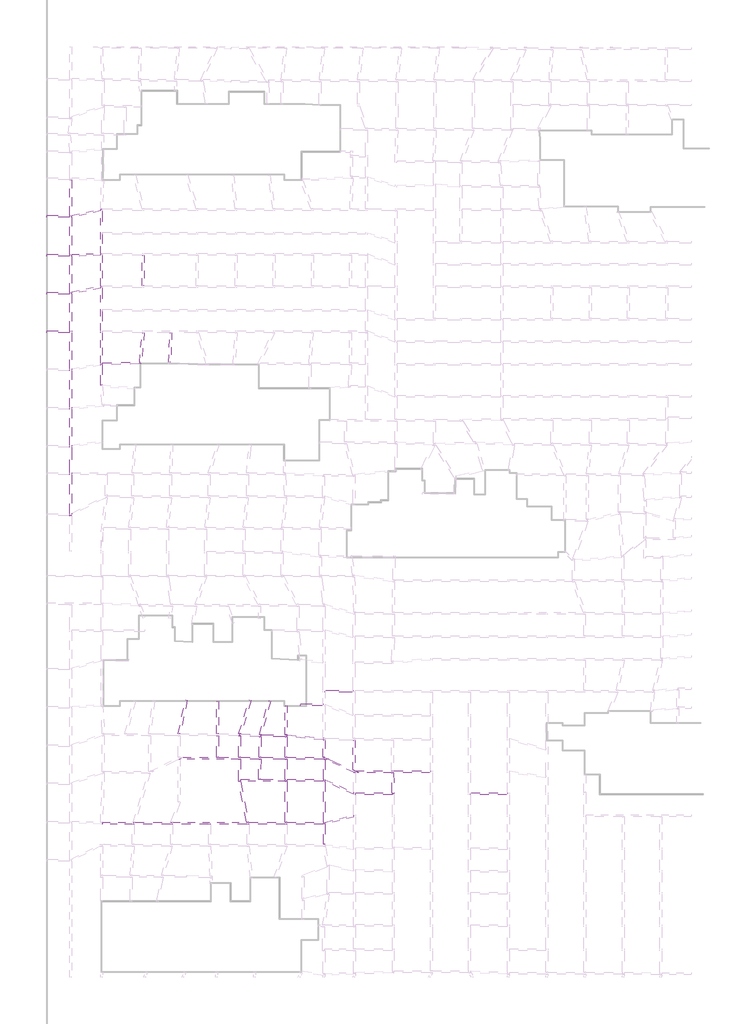
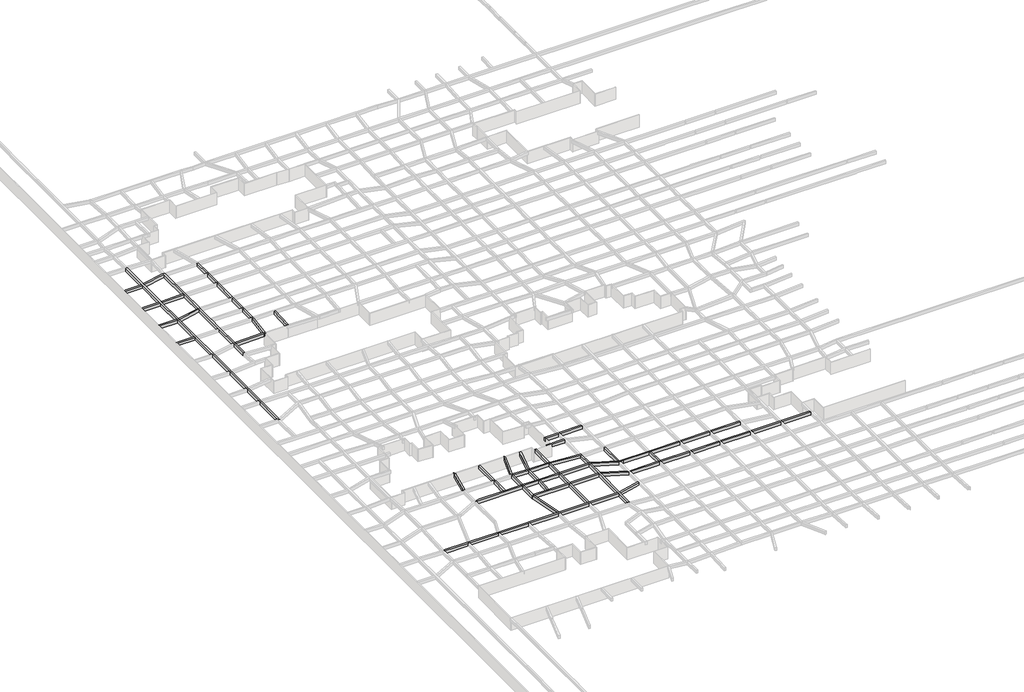
# One storey, part 26 of 45: 46 beams.
"""IFC4 building model written with IfcOpenShell, lengths in millimetres."""

from ifc_helpers import new_model, si_unit, frame, origin, place, context, project, spatial, polyline, outline, extrude, faceted_brep, element, save

model = new_model("IFC4")

# Units and contexts
model_context = context("Model", 3, world=origin())
ifc_project = project(units=[si_unit("LENGTHUNIT", "METRE", prefix="MILLI")], contexts=[model_context])

# Site, building, storey
site = spatial("IfcSite", under=ifc_project)
building = spatial("IfcBuilding", under=site)
storey = spatial("IfcBuildingStorey", under=building, Name="户型图", Elevation=0.0)

# Beams
placement = place(None, origin())
element("IfcBeam", 1, ObjectType="混凝土 - 矩形梁 : KL_beam", at=placement, inside=storey, context=model_context, shape_type="Brep", body=[
    faceted_brep([(-150359.8528414, 63929.9626201, 3300.0), (-150112.1714971, 63929.9626201, 3300.0), (-149959.8528414, 63929.9626201, 3300.0), (-149959.8528414, 64007.5728516, 3300.0), (-149959.8528414, 64456.5033467, 3300.0), (-149959.8528414, 72229.932653, 3300.0), (-149959.8528414, 72629.932653, 3300.0), (-149959.8528414, 77856.1223033, 3300.0), (-149959.8528414, 78260.0533323, 3300.0), (-149959.8528414, 85546.6664182, 3300.0), (-149959.8528414, 85948.1943532, 3300.0), (-149959.8528414, 93365.130378, 3300.0), (-149959.8528414, 93772.617056, 3300.0), (-149959.8528414, 101129.932653, 3300.0), (-149959.8528414, 101529.932653, 3300.0), (-149959.8528414, 108967.3783069, 3300.0), (-149959.8528414, 109376.0042036, 3300.0), (-149959.8528414, 116635.7245612, 3300.0), (-149959.8528414, 117035.8972944, 3300.0), (-149959.8528414, 124568.9031862, 3300.0), (-149959.8528414, 124978.3343946, 3300.0), (-149959.8528414, 132222.8565574, 3300.0), (-150162.4857077, 132229.932653, 3300.0), (-150359.8528414, 132229.932653, 3300.0), (-150359.8528414, 124929.932653, 3300.0), (-150359.8528414, 124529.932653, 3300.0), (-150359.8528414, 117029.932653, 3300.0), (-150359.8528414, 116629.932653, 3300.0), (-150359.8528414, 109329.932653, 3300.0), (-150359.8528414, 108929.932653, 3300.0), (-150359.8528414, 101529.932653, 3300.0), (-150359.8528414, 101129.932653, 3300.0), (-150359.8528414, 93729.932653, 3300.0), (-150359.8528414, 93329.932653, 3300.0), (-150359.8528414, 85929.932653, 3300.0), (-150359.8528414, 85529.932653, 3300.0), (-150359.8528414, 78229.932653, 3300.0), (-150359.8528414, 77829.932653, 3300.0), (-150359.8528414, 72629.932653, 3300.0), (-150359.8528414, 72229.932653, 3300.0), (-150359.8528414, 64329.9626201, 3300.0), (-150359.8528414, 63929.9626201, 2500.0), (-150359.8528414, 132229.932653, 2500.0), (-150359.8528414, 124929.932653, 2500.0), (-150359.8528414, 124529.932653, 2500.0), (-150359.8528414, 117029.932653, 2500.0), (-150359.8528414, 116629.932653, 2500.0), (-150359.8528414, 109329.932653, 2500.0), (-150359.8528414, 108929.932653, 2500.0), (-150359.8528414, 101529.932653, 2500.0), (-150359.8528414, 101129.932653, 2500.0), (-150359.8528414, 93729.932653, 2500.0), (-150359.8528414, 93329.932653, 2500.0), (-150359.8528414, 85929.932653, 2500.0), (-150359.8528414, 85529.932653, 2500.0), (-150359.8528414, 78229.932653, 2500.0), (-150359.8528414, 77829.932653, 2500.0), (-150359.8528414, 72629.932653, 2500.0), (-150359.8528414, 72229.932653, 2500.0), (-150359.8528414, 64329.9626201, 2500.0), (-149959.8528414, 63929.9626201, 2500.0), (-150112.1714971, 63929.9626201, 2500.0), (-150162.4857077, 132229.932653, 2500.0), (-149959.8528414, 132222.8565574, 2500.0), (-149959.8528414, 124978.3343946, 2500.0), (-149959.8528414, 124568.9031862, 2500.0), (-149959.8528414, 117035.8972944, 2500.0), (-149959.8528414, 116635.7245612, 2500.0), (-149959.8528414, 109376.0042036, 2500.0), (-149959.8528414, 108967.3783069, 2500.0), (-149959.8528414, 101529.932653, 2500.0), (-149959.8528414, 101129.932653, 2500.0), (-149959.8528414, 93772.617056, 2500.0), (-149959.8528414, 93365.130378, 2500.0), (-149959.8528414, 85948.1943532, 2500.0), (-149959.8528414, 85546.6664182, 2500.0), (-149959.8528414, 78260.0533323, 2500.0), (-149959.8528414, 77856.1223033, 2500.0), (-149959.8528414, 72629.932653, 2500.0), (-149959.8528414, 72229.932653, 2500.0), (-149959.8528414, 64456.5033467, 2500.0), (-149959.8528414, 64007.5728516, 2500.0)], [[[0, 1, 2, 3, 4, 5, 6, 7, 8, 9, 10, 11, 12, 13, 14, 15, 16, 17, 18, 19, 20, 21, 22, 23, 24, 25, 26, 27, 28, 29, 30, 31, 32, 33, 34, 35, 36, 37, 38, 39, 40]], [[41, 0, 40, 39, 38, 37, 36, 35, 34, 33, 32, 31, 30, 29, 28, 27, 26, 25, 24, 23, 42, 43, 44, 45, 46, 47, 48, 49, 50, 51, 52, 53, 54, 55, 56, 57, 58, 59]], [[60, 61, 41, 59, 58, 57, 56, 55, 54, 53, 52, 51, 50, 49, 48, 47, 46, 45, 44, 43, 42, 62, 63, 64, 65, 66, 67, 68, 69, 70, 71, 72, 73, 74, 75, 76, 77, 78, 79, 80, 81]], [[63, 21, 20, 19, 18, 17, 16, 15, 14, 13, 12, 11, 10, 9, 8, 7, 6, 5, 4, 3, 2, 60, 81, 80, 79, 78, 77, 76, 75, 74, 73, 72, 71, 70, 69, 68, 67, 66, 65, 64]], [[21, 63, 62, 22]], [[23, 22, 62, 42]], [[2, 1, 0, 41, 61, 60]]]),
])
element("IfcBeam", 2, ObjectType="混凝土 - 矩形梁 : KL_beam", at=placement, inside=storey, context=model_context, shape_type="SweptSolid", body=[
    extrude(outline(polyline([(-155040.1872489, 124529.932653), (-155040.1872489, 124929.932653), (-150359.8528414, 124929.932653), (-150359.8528414, 124529.932653), (-155040.1872489, 124529.932653)])), frame((0.0, 0.0, 2500.0), z_axis=(0.0, 0.0, 1.0), x_axis=(1.0, 0.0, 0.0)), (0.0, 0.0, 1.0), 800.0),
])
element("IfcBeam", 3, ObjectType="混凝土 - 矩形梁 : KL_beam", at=placement, inside=storey, context=model_context, shape_type="SweptSolid", body=[
    extrude(outline(polyline([(-155040.1872489, 116629.932653), (-155040.1872489, 117029.932653), (-150359.8528414, 117029.932653), (-150359.8528414, 116629.932653), (-155040.1872489, 116629.932653)])), frame((0.0, 0.0, 2500.0), z_axis=(0.0, 0.0, 1.0), x_axis=(1.0, 0.0, 0.0)), (0.0, 0.0, 1.0), 800.0),
])
element("IfcBeam", 4, ObjectType="混凝土 - 矩形梁 : KL_beam", at=placement, inside=storey, context=model_context, shape_type="SweptSolid", body=[
    extrude(outline(polyline([(-155040.1872489, 108929.932653), (-155040.1872489, 109329.932653), (-150359.8528414, 109329.932653), (-150359.8528414, 108929.932653), (-155040.1872489, 108929.932653)])), frame((0.0, 0.0, 2500.0), z_axis=(0.0, 0.0, 1.0), x_axis=(1.0, 0.0, 0.0)), (0.0, 0.0, 1.0), 800.0),
])
element("IfcBeam", 5, ObjectType="混凝土 - 矩形梁 : KL_beam", at=placement, inside=storey, context=model_context, shape_type="SweptSolid", body=[
    extrude(outline(polyline([(-155040.1872489, 101129.932653), (-155040.1872489, 101529.932653), (-150359.8528414, 101529.932653), (-150359.8528414, 101129.932653), (-155040.1872489, 101129.932653)])), frame((0.0, 0.0, 2500.0), z_axis=(0.0, 0.0, 1.0), x_axis=(1.0, 0.0, 0.0)), (0.0, 0.0, 1.0), 800.0),
])
element("IfcBeam", 6, ObjectType="混凝土 - 矩形梁 : KL_beam", at=placement, inside=storey, context=model_context, shape_type="Brep", body=[
    faceted_brep([(-144133.590805, 126250.9688143, 3300.0), (-144133.590805, 125841.5376059, 3300.0), (-144133.590805, 117207.1391417, 3300.0), (-144133.590805, 116806.9664084, 3300.0), (-144133.590805, 110592.4869991, 3300.0), (-144133.590805, 110183.8611024, 3300.0), (-144133.590805, 101529.932653, 3300.0), (-144133.590805, 101129.932653, 3300.0), (-144133.590805, 94905.1276718, 3300.0), (-144133.590805, 94497.6409938, 3300.0), (-144133.590805, 90443.9102418, 3300.0), (-143749.2394727, 90477.5366261, 3300.0), (-143733.590805, 90476.4423647, 3300.0), (-143733.590805, 94545.5936478, 3300.0), (-143733.590805, 94945.7388373, 3300.0), (-143733.590805, 101129.932653, 3300.0), (-143733.590805, 101529.932653, 3300.0), (-143733.590805, 105423.4823743, 3300.0), (-143733.590805, 105823.4823743, 3300.0), (-143733.590805, 110229.932653, 3300.0), (-143733.590805, 110629.932653, 3300.0), (-143733.590805, 116812.9362228, 3300.0), (-143733.590805, 117212.9362228, 3300.0), (-143733.590805, 121089.9393475, 3300.0), (-143733.590805, 121489.9393475, 3300.0), (-143733.590805, 125889.9393475, 3300.0), (-143733.590805, 126001.9198071, 3300.0), (-143733.590805, 126250.9688143, 3300.0), (-144087.2760394, 126250.9688143, 3300.0), (-143733.590805, 126250.9688143, 2500.0), (-143733.590805, 90476.4423647, 2500.0), (-143733.590805, 94545.5936478, 2500.0), (-143733.590805, 94945.7388373, 2500.0), (-143733.590805, 101129.932653, 2500.0), (-143733.590805, 101529.932653, 2500.0), (-143733.590805, 105423.4823743, 2500.0), (-143733.590805, 105823.4823743, 2500.0), (-143733.590805, 110229.932653, 2500.0), (-143733.590805, 110629.932653, 2500.0), (-143733.590805, 116812.9362228, 2500.0), (-143733.590805, 117212.9362228, 2500.0), (-143733.590805, 121089.9393475, 2500.0), (-143733.590805, 121489.9393475, 2500.0), (-143733.590805, 125889.9393475, 2500.0), (-143733.590805, 126001.9198071, 2500.0), (-144133.590805, 90443.9102418, 2500.0), (-144133.590805, 94497.6409938, 2500.0), (-144133.590805, 94905.1276718, 2500.0), (-144133.590805, 101129.932653, 2500.0), (-144133.590805, 101529.932653, 2500.0), (-144133.590805, 110183.8611024, 2500.0), (-144133.590805, 110592.4869991, 2500.0), (-144133.590805, 116806.9664084, 2500.0), (-144133.590805, 117207.1391417, 2500.0), (-144133.590805, 125841.5376059, 2500.0), (-144133.590805, 126250.9688143, 2500.0), (-144087.2760394, 126250.9688143, 2500.0), (-143749.2394727, 90477.5366261, 2500.0)], [[[0, 1, 2, 3, 4, 5, 6, 7, 8, 9, 10, 11, 12, 13, 14, 15, 16, 17, 18, 19, 20, 21, 22, 23, 24, 25, 26, 27, 28]], [[29, 27, 26, 25, 24, 23, 22, 21, 20, 19, 18, 17, 16, 15, 14, 13, 12, 30, 31, 32, 33, 34, 35, 36, 37, 38, 39, 40, 41, 42, 43, 44]], [[45, 46, 47, 48, 49, 50, 51, 52, 53, 54, 55, 56, 29, 44, 43, 42, 41, 40, 39, 38, 37, 36, 35, 34, 33, 32, 31, 30, 57]], [[10, 9, 8, 7, 6, 5, 4, 3, 2, 1, 0, 55, 54, 53, 52, 51, 50, 49, 48, 47, 46, 45]], [[11, 10, 45, 57]], [[12, 11, 57, 30]], [[0, 28, 27, 29, 56, 55]]]),
])
element("IfcBeam", 7, ObjectType="混凝土 - 矩形梁 : KL_beam", at=placement, inside=storey, context=model_context, shape_type="SweptSolid", body=[
    extrude(outline(polyline([(-144133.590805, 126250.9688143), (-144133.590805, 125841.5376059), (-149959.8528414, 124568.9031862), (-149959.8528414, 124978.3343946), (-144133.590805, 126250.9688143)])), frame((0.0, 0.0, 2500.0), z_axis=(0.0, 0.0, 1.0), x_axis=(1.0, 0.0, 0.0)), (0.0, 0.0, 1.0), 800.0),
])
element("IfcBeam", 8, ObjectType="混凝土 - 矩形梁 : KL_beam", at=placement, inside=storey, context=model_context, shape_type="SweptSolid", body=[
    extrude(outline(polyline([(-135233.590805, 101529.932653), (-135633.590805, 101529.932653), (-135633.590805, 105423.4823743), (-135233.590805, 105423.4823743), (-135233.590805, 101529.932653)])), frame((0.0, 0.0, 2500.0), z_axis=(0.0, 0.0, 1.0), x_axis=(1.0, 0.0, 0.0)), (0.0, 0.0, 1.0), 800.0),
    extrude(outline(polyline([(-135633.590805, 125889.9393475), (-135233.590805, 125889.9393475), (-135233.590805, 121489.9393475), (-135633.590805, 121489.9393475), (-135633.590805, 125889.9393475)])), frame((0.0, 0.0, 2500.0), z_axis=(0.0, 0.0, 1.0), x_axis=(1.0, 0.0, 0.0)), (0.0, 0.0, 1.0), 800.0),
    extrude(outline(polyline([(-135633.590805, 121089.9393475), (-135233.590805, 121089.9393475), (-135233.590805, 117212.9362228), (-135633.590805, 117212.9362228), (-135633.590805, 121089.9393475)])), frame((0.0, 0.0, 2500.0), z_axis=(0.0, 0.0, 1.0), x_axis=(1.0, 0.0, 0.0)), (0.0, 0.0, 1.0), 800.0),
    extrude(outline(polyline([(-135633.590805, 116812.9362228), (-135233.590805, 116812.9362228), (-135233.590805, 110629.932653), (-135633.590805, 110629.932653), (-135633.590805, 116812.9362228)])), frame((0.0, 0.0, 2500.0), z_axis=(0.0, 0.0, 1.0), x_axis=(1.0, 0.0, 0.0)), (0.0, 0.0, 1.0), 800.0),
    extrude(outline(polyline([(-135633.590805, 110229.932653), (-135233.590805, 110229.932653), (-135233.590805, 105823.4823743), (-135633.590805, 105823.4823743), (-135633.590805, 110229.932653)])), frame((0.0, 0.0, 2500.0), z_axis=(0.0, 0.0, 1.0), x_axis=(1.0, 0.0, 0.0)), (0.0, 0.0, 1.0), 800.0),
])
element("IfcBeam", 9, ObjectType="混凝土 - 矩形梁 : KL_beam", at=placement, inside=storey, context=model_context, shape_type="SweptSolid", body=[
    extrude(outline(polyline([(-149959.8528414, 108967.3783069), (-149959.8528414, 109376.0042036), (-144133.590805, 110592.4869991), (-144133.590805, 110183.8611024), (-149959.8528414, 108967.3783069)])), frame((0.0, 0.0, 2500.0), z_axis=(0.0, 0.0, 1.0), x_axis=(1.0, 0.0, 0.0)), (0.0, 0.0, 1.0), 800.0),
])
element("IfcBeam", 10, ObjectType="混凝土 - 矩形梁 : KL_beam", at=placement, inside=storey, context=model_context, shape_type="SweptSolid", body=[
    extrude(outline(polyline([(-149959.8528414, 116635.7245612), (-149959.8528414, 117035.8972944), (-144133.590805, 117207.1391417), (-144133.590805, 116806.9664084), (-149959.8528414, 116635.7245612)])), frame((0.0, 0.0, 2500.0), z_axis=(0.0, 0.0, 1.0), x_axis=(1.0, 0.0, 0.0)), (0.0, 0.0, 1.0), 800.0),
])
element("IfcBeam", 11, ObjectType="混凝土 - 矩形梁 : KL_beam", at=placement, inside=storey, context=model_context, shape_type="SweptSolid", body=[
    extrude(outline(polyline([(-129850.782274, 95106.8917227), (-130250.5386048, 95120.8515214), (-130040.6968677, 101129.932653), (-129640.45305, 101129.932653), (-129850.782274, 95106.8917227)])), frame((0.0, 0.0, 2500.0), z_axis=(0.0, 0.0, 1.0), x_axis=(1.0, 0.0, 0.0)), (0.0, 0.0, 1.0), 800.0),
])
element("IfcBeam", 12, ObjectType="混凝土 - 矩形梁 : KL_beam", at=placement, inside=storey, context=model_context, shape_type="Brep", body=[
    faceted_brep([(-136210.1713836, 94748.3186716, 3300.0), (-135807.6946267, 94759.1637549, 3300.0), (-135250.3245702, 101129.932653, 3300.0), (-135651.8525052, 101129.932653, 3300.0), (-136175.0804904, 95149.4094155, 3300.0), (-136210.1713836, 94748.3186716, 2500.0), (-135651.8525052, 101129.932653, 2500.0), (-136175.0804904, 95149.4094155, 2500.0), (-135807.6946267, 94759.1637549, 2500.0), (-135250.3245702, 101129.932653, 2500.0)], [[[0, 1, 2, 3, 4]], [[5, 0, 4, 3, 6, 7]], [[8, 5, 7, 6, 9]], [[1, 8, 9, 2]], [[3, 2, 9, 6]], [[1, 0, 5, 8]]]),
])
element("IfcBeam", 13, ObjectType="混凝土 - 矩形梁 : KL_beam", at=placement, inside=storey, context=model_context, shape_type="SweptSolid", body=[
    extrude(outline(polyline([(-136175.0804904, 95149.4094155), (-136210.1713836, 94748.3186716), (-143733.590805, 94545.5936478), (-143733.590805, 94945.7388373), (-136175.0804904, 95149.4094155)])), frame((0.0, 0.0, 2500.0), z_axis=(0.0, 0.0, 1.0), x_axis=(1.0, 0.0, 0.0)), (0.0, 0.0, 1.0), 800.0),
])
element("IfcBeam", 14, ObjectType="混凝土 - 矩形梁 : KL_beam", at=placement, inside=storey, context=model_context, shape_type="Brep", body=[
    faceted_brep([(-115838.9400314, 19632.6251957, 3300.0), (-115849.4144, 19232.6251957, 3300.0), (-115644.2371144, 19221.8723098, 3300.0), (-111849.9331697, 19023.0212661, 3300.0), (-111449.9331697, 19002.0581544, 3300.0), (-111449.9331697, 19012.5835366, 3300.0), (-111449.9331697, 19402.6070928, 3300.0), (-111640.2950559, 19412.5835366, 3300.0), (-111801.1398842, 19421.0130568, 3300.0), (-115578.0725211, 19618.9537088, 3300.0), (-115849.4144, 19232.6251957, 2500.0), (-115644.2371144, 19221.8723098, 2500.0), (-111849.9331697, 19023.0212661, 2500.0), (-111449.9331697, 19002.0581544, 2500.0), (-115838.9400314, 19632.6251957, 2500.0), (-115578.0725211, 19618.9537088, 2500.0), (-111801.1398842, 19421.0130568, 2500.0), (-111640.2950559, 19412.5835366, 2500.0), (-111449.9331697, 19402.6070928, 2500.0), (-111449.9331697, 19012.5835366, 2500.0)], [[[0, 1, 2, 3, 4, 5, 6, 7, 8, 9]], [[1, 10, 11, 12, 13, 4, 3, 2]], [[10, 14, 15, 16, 17, 18, 19, 13, 12, 11]], [[14, 0, 9, 8, 7, 6, 18, 17, 16, 15]], [[0, 14, 10, 1]], [[6, 5, 4, 13, 19, 18]]]),
])
element("IfcBeam", 15, ObjectType="混凝土 - 矩形梁 : KL_beam", at=placement, inside=storey, context=model_context, shape_type="Brep", body=[
    faceted_brep([(-97671.9511598, 14425.3528936, 3300.0), (-98434.5356576, 14764.877387, 3300.0), (-98570.3658693, 14825.3528936, 3300.0), (-98834.5356576, 14825.3528936, 3300.0), (-106149.9331697, 14825.3528936, 3300.0), (-106549.9331697, 14825.3528936, 3300.0), (-111449.9331697, 14825.3528936, 3300.0), (-111849.9331697, 14825.3528936, 3300.0), (-115644.2371144, 14825.3528936, 3300.0), (-116044.2371144, 14825.3528936, 3300.0), (-120144.2950634, 14825.3528936, 3300.0), (-120544.2950634, 14825.3528936, 3300.0), (-127346.5820068, 14825.3528936, 3300.0), (-128166.7035435, 14425.3528936, 3300.0), (-127944.2950634, 14425.3528936, 3300.0), (-116044.2371144, 14425.3528936, 3300.0), (-115644.2371144, 14425.3528936, 3300.0), (-111857.0472867, 14425.3528936, 3300.0), (-111456.803469, 14425.3528936, 3300.0), (-106549.9331697, 14425.3528936, 3300.0), (-106149.9331697, 14425.3528936, 3300.0), (-98812.8771817, 14425.3528936, 3300.0), (-98655.388494, 14425.3528936, 3300.0), (-97671.9511598, 14425.3528936, 2500.0), (-128166.7035435, 14425.3528936, 2500.0), (-127944.2950634, 14425.3528936, 2500.0), (-116044.2371144, 14425.3528936, 2500.0), (-115644.2371144, 14425.3528936, 2500.0), (-111857.0472867, 14425.3528936, 2500.0), (-111456.803469, 14425.3528936, 2500.0), (-106549.9331697, 14425.3528936, 2500.0), (-106149.9331697, 14425.3528936, 2500.0), (-98812.8771817, 14425.3528936, 2500.0), (-98655.388494, 14425.3528936, 2500.0), (-98570.3658693, 14825.3528936, 2500.0), (-98434.5356576, 14764.877387, 2500.0), (-127346.5820068, 14825.3528936, 2500.0), (-120544.2950634, 14825.3528936, 2500.0), (-120144.2950634, 14825.3528936, 2500.0), (-116044.2371144, 14825.3528936, 2500.0), (-115644.2371144, 14825.3528936, 2500.0), (-111849.9331697, 14825.3528936, 2500.0), (-111449.9331697, 14825.3528936, 2500.0), (-106549.9331697, 14825.3528936, 2500.0), (-106149.9331697, 14825.3528936, 2500.0), (-98834.5356576, 14825.3528936, 2500.0)], [[[0, 1, 2, 3, 4, 5, 6, 7, 8, 9, 10, 11, 12, 13, 14, 15, 16, 17, 18, 19, 20, 21, 22]], [[23, 0, 22, 21, 20, 19, 18, 17, 16, 15, 14, 13, 24, 25, 26, 27, 28, 29, 30, 31, 32, 33]], [[34, 35, 23, 33, 32, 31, 30, 29, 28, 27, 26, 25, 24, 36, 37, 38, 39, 40, 41, 42, 43, 44, 45]], [[2, 34, 45, 44, 43, 42, 41, 40, 39, 38, 37, 36, 12, 11, 10, 9, 8, 7, 6, 5, 4, 3]], [[13, 12, 36, 24]], [[2, 1, 0, 23, 35, 34]]]),
])
element("IfcBeam", 16, ObjectType="混凝土 - 矩形梁 : KL_beam", at=placement, inside=storey, context=model_context, shape_type="SweptSolid", body=[
    extrude(outline(polyline([(-120544.2950634, 19232.6251957), (-120144.2950634, 19232.6251957), (-120144.2950634, 14825.3528936), (-120544.2950634, 14825.3528936), (-120544.2950634, 19232.6251957)])), frame((0.0, 0.0, 2500.0), z_axis=(0.0, 0.0, 1.0), x_axis=(1.0, 0.0, 0.0)), (0.0, 0.0, 1.0), 800.0),
])
element("IfcBeam", 17, ObjectType="混凝土 - 矩形梁 : KL_beam", at=placement, inside=storey, context=model_context, shape_type="SweptSolid", body=[
    extrude(outline(polyline([(-115644.2371144, 14825.3528936), (-116044.2371144, 14825.3528936), (-116044.2371144, 19232.6251957), (-115849.4144, 19232.6251957), (-115644.2371144, 19221.8723098), (-115644.2371144, 14825.3528936)])), frame((0.0, 0.0, 2500.0), z_axis=(0.0, 0.0, 1.0), x_axis=(1.0, 0.0, 0.0)), (0.0, 0.0, 1.0), 800.0),
])
element("IfcBeam", 18, ObjectType="混凝土 - 矩形梁 : KL_beam", at=placement, inside=storey, context=model_context, shape_type="SweptSolid", body=[
    extrude(outline(polyline([(-111849.9331697, 19023.0212661), (-111449.9331697, 19002.0581544), (-111449.9331697, 14825.3528936), (-111849.9331697, 14825.3528936), (-111849.9331697, 19023.0212661)])), frame((0.0, 0.0, 2500.0), z_axis=(0.0, 0.0, 1.0), x_axis=(1.0, 0.0, 0.0)), (0.0, 0.0, 1.0), 800.0),
])
element("IfcBeam", 19, ObjectType="混凝土 - 矩形梁 : KL_beam", at=placement, inside=storey, context=model_context, shape_type="Brep", body=[
    faceted_brep([(-111449.9331697, 19402.6070928, 3300.0), (-111449.9331697, 19012.5835366, 3300.0), (-106549.9331697, 19012.5835366, 3300.0), (-106149.9331697, 19012.5835366, 3300.0), (-106149.9331697, 19395.8497714, 3300.0), (-106149.9331697, 19412.5835366, 3300.0), (-106341.2009811, 19412.5835366, 3300.0), (-106549.9331697, 19412.5835366, 3300.0), (-111389.2880952, 19412.5835366, 3300.0), (-111640.2950559, 19412.5835366, 3300.0), (-111449.9331697, 19012.5835366, 2500.0), (-106549.9331697, 19012.5835366, 2500.0), (-106149.9331697, 19012.5835366, 2500.0), (-111449.9331697, 19402.6070928, 2500.0), (-111640.2950559, 19412.5835366, 2500.0), (-111389.2880952, 19412.5835366, 2500.0), (-106549.9331697, 19412.5835366, 2500.0), (-106341.2009811, 19412.5835366, 2500.0), (-106149.9331697, 19412.5835366, 2500.0), (-106149.9331697, 19395.8497714, 2500.0)], [[[0, 1, 2, 3, 4, 5, 6, 7, 8, 9]], [[1, 10, 11, 12, 3, 2]], [[10, 13, 14, 15, 16, 17, 18, 19, 12, 11]], [[14, 9, 8, 7, 6, 5, 18, 17, 16, 15]], [[0, 13, 10, 1]], [[13, 0, 9, 14]], [[5, 4, 3, 12, 19, 18]]]),
])
element("IfcBeam", 20, ObjectType="混凝土 - 矩形梁 : KL_beam", at=placement, inside=storey, context=model_context, shape_type="Brep", body=[
    faceted_brep([(-106149.9331697, 19012.5835366, 3300.0), (-106549.9331697, 19012.5835366, 3300.0), (-106549.9331697, 14825.3528936, 3300.0), (-106149.9331697, 14825.3528936, 3300.0), (-106149.9331697, 18994.3218363, 3300.0), (-106549.9331697, 19012.5835366, 2500.0), (-106549.9331697, 14825.3528936, 2500.0), (-106149.9331697, 19012.5835366, 2500.0), (-106149.9331697, 18994.3218363, 2500.0), (-106149.9331697, 14825.3528936, 2500.0)], [[[0, 1, 2, 3, 4]], [[1, 5, 6, 2]], [[5, 7, 8, 9, 6]], [[7, 0, 4, 3, 9, 8]], [[1, 0, 7, 5]], [[3, 2, 6, 9]]]),
])
element("IfcBeam", 21, ObjectType="混凝土 - 矩形梁 : KL_beam", at=placement, inside=storey, context=model_context, shape_type="Brep", body=[
    faceted_brep([(-106341.2009811, 19412.5835366, 3300.0), (-106549.9331697, 19430.8452368, 3300.0), (-106549.9331697, 19412.5835366, 3300.0), (-106549.9331697, 19430.8452368, 2500.0), (-106341.2009811, 19412.5835366, 2500.0), (-106549.9331697, 19412.5835366, 2500.0)], [[[0, 1, 2]], [[3, 4, 5]], [[1, 0, 4, 3]], [[5, 2, 1, 3]], [[0, 2, 5, 4]]]),
    faceted_brep([(-98447.5025342, 18320.4464741, 2500.0), (-98447.5025342, 18320.4464741, 3300.0), (-98834.5356576, 18354.3074848, 3300.0), (-106149.9331697, 18994.3218363, 3300.0), (-106149.9331697, 18994.3218363, 2500.0), (-98834.5356576, 18354.3074848, 2500.0), (-106149.9331697, 19395.8497714, 3300.0), (-106149.9331697, 19395.8497714, 2500.0), (-106149.9331697, 19012.5835366, 2500.0), (-106149.9331697, 19012.5835366, 3300.0), (-98430.038157, 18720.4464741, 3300.0), (-98430.038157, 18720.4464741, 2500.0), (-98434.5356576, 18720.8399544, 3300.0), (-98834.5356576, 18755.8354199, 3300.0), (-98834.5356576, 18755.8354199, 2500.0), (-98434.5356576, 18720.8399544, 2500.0)], [[[0, 1, 2, 3, 4, 5]], [[6, 7, 8, 4, 3, 9]], [[10, 1, 0, 11]], [[6, 9, 3, 2, 1, 10, 12, 13]], [[4, 8, 7, 14, 15, 11, 0, 5]], [[7, 6, 13, 12, 10, 11, 15, 14]]]),
])
element("IfcBeam", 22, ObjectType="混凝土 - 矩形梁 : KL_beam", at=placement, inside=storey, context=model_context, shape_type="Brep", body=[
    faceted_brep([(-92534.6339278, 11700.217385, 3300.0), (-92291.6701424, 11700.217385, 3300.0), (-91551.1965936, 11700.217385, 3300.0), (-92449.6113031, 12100.217385, 3300.0), (-92755.3337307, 12236.3337795, 3300.0), (-97671.9511598, 14425.3528936, 3300.0), (-98655.388494, 14425.3528936, 3300.0), (-98412.8771817, 14317.3799008, 3300.0), (-92691.6701424, 11770.1344124, 3300.0), (-92534.6339278, 11700.217385, 2500.0), (-98655.388494, 14425.3528936, 2500.0), (-98412.8771817, 14317.3799008, 2500.0), (-92691.6701424, 11770.1344124, 2500.0), (-91551.1965936, 11700.217385, 2500.0), (-92291.6701424, 11700.217385, 2500.0), (-97671.9511598, 14425.3528936, 2500.0), (-92755.3337307, 12236.3337795, 2500.0), (-92449.6113031, 12100.217385, 2500.0)], [[[0, 1, 2, 3, 4, 5, 6, 7, 8]], [[9, 0, 8, 7, 6, 10, 11, 12]], [[13, 14, 9, 12, 11, 10, 15, 16, 17]], [[2, 13, 17, 16, 15, 5, 4, 3]], [[6, 5, 15, 10]], [[2, 1, 0, 9, 14, 13]]]),
])
element("IfcBeam", 23, ObjectType="混凝土 - 矩形梁 : KL_beam", at=placement, inside=storey, context=model_context, shape_type="Brep", body=[
    faceted_brep([(-61385.2176693, 11700.217385, 3300.0), (-61385.2176693, 12100.217385, 3300.0), (-68859.410716, 12100.217385, 3300.0), (-68859.410716, 11700.217385, 3300.0), (-61385.2176693, 11700.217385, 2500.0), (-68859.410716, 11700.217385, 2500.0), (-61385.2176693, 12100.217385, 2500.0), (-68859.410716, 12100.217385, 2500.0)], [[[0, 1, 2, 3]], [[4, 0, 3, 5]], [[6, 4, 5, 7]], [[1, 6, 7, 2]], [[1, 0, 4, 6]], [[3, 2, 7, 5]]]),
    faceted_brep([(-91551.1965936, 11700.217385, 3300.0), (-92449.6113031, 12100.217385, 3300.0), (-92449.6113031, 12100.217385, 2500.0), (-91551.1965936, 11700.217385, 2500.0), (-76974.0592951, 12100.217385, 3300.0), (-76974.0592951, 11700.217385, 3300.0), (-76974.0592951, 11700.217385, 2500.0), (-76974.0592951, 12100.217385, 2500.0), (-84936.5912928, 11700.217385, 3300.0), (-84536.3474751, 11700.217385, 3300.0), (-84543.4535378, 12100.217385, 3300.0), (-84943.4535378, 12100.217385, 3300.0), (-92355.3337307, 12100.217385, 3300.0), (-84936.5912928, 11700.217385, 2500.0), (-84536.3474751, 11700.217385, 2500.0), (-92355.3337307, 12100.217385, 2500.0), (-84943.4535378, 12100.217385, 2500.0), (-84543.4535378, 12100.217385, 2500.0)], [[[0, 1, 2, 3]], [[4, 5, 6, 7]], [[1, 0, 8, 9, 5, 4, 10, 11, 12]], [[0, 3, 13, 14, 6, 5, 9, 8]], [[3, 2, 15, 16, 17, 7, 6, 14, 13]], [[2, 1, 12, 11, 10, 4, 7, 17, 16, 15]]]),
    faceted_brep([(-76574.0592951, 11700.217385, 3300.0), (-76574.0592951, 12100.217385, 3300.0), (-76574.0592951, 12100.217385, 2500.0), (-76574.0592951, 11700.217385, 2500.0), (-69259.410716, 12100.217385, 3300.0), (-69259.410716, 11700.217385, 3300.0), (-69259.410716, 11700.217385, 2500.0), (-69259.410716, 12100.217385, 2500.0)], [[[0, 1, 2, 3]], [[4, 5, 6, 7]], [[1, 0, 5, 4]], [[0, 3, 6, 5]], [[3, 2, 7, 6]], [[2, 1, 4, 7]]]),
])
element("IfcBeam", 24, ObjectType="混凝土 - 矩形梁 : KL_beam", at=placement, inside=storey, context=model_context, shape_type="SweptSolid", body=[
    extrude(outline(polyline([(-92691.6701424, 7708.1903778), (-92691.6701424, 7270.3358664), (-98412.8771817, 9817.5813548), (-98412.8771817, 10255.4358662), (-92691.6701424, 7708.1903778)])), frame((0.0, 0.0, 2500.0), z_axis=(0.0, 0.0, 1.0), x_axis=(1.0, 0.0, 0.0)), (0.0, 0.0, 1.0), 800.0),
])
element("IfcBeam", 25, ObjectType="混凝土 - 矩形梁 : KL_beam", at=placement, inside=storey, context=model_context, shape_type="Brep", body=[
    faceted_brep([(-98812.8771817, -2906.533538, 3300.0), (-98412.8771817, -2906.533538, 3300.0), (-98412.8771817, 1237.2093367, 3300.0), (-98412.8771817, 1649.4547885, 3300.0), (-98412.8771817, 9817.5813548, 3300.0), (-98412.8771817, 10255.4358662, 3300.0), (-98412.8771817, 14317.3799008, 3300.0), (-98655.388494, 14425.3528936, 3300.0), (-98812.8771817, 14425.3528936, 3300.0), (-98812.8771817, 10325.4890447, 3300.0), (-98812.8771817, 9925.4890447, 3300.0), (-98812.8771817, 1593.466462, 3300.0), (-98812.8771817, 1193.466462, 3300.0), (-98812.8771817, -2906.533538, 2500.0), (-98812.8771817, 14425.3528936, 2500.0), (-98812.8771817, 10325.4890447, 2500.0), (-98812.8771817, 9925.4890447, 2500.0), (-98812.8771817, 1593.466462, 2500.0), (-98812.8771817, 1193.466462, 2500.0), (-98412.8771817, -2906.533538, 2500.0), (-98655.388494, 14425.3528936, 2500.0), (-98412.8771817, 14317.3799008, 2500.0), (-98412.8771817, 10255.4358662, 2500.0), (-98412.8771817, 9817.5813548, 2500.0), (-98412.8771817, 1649.4547885, 2500.0), (-98412.8771817, 1237.2093367, 2500.0)], [[[0, 1, 2, 3, 4, 5, 6, 7, 8, 9, 10, 11, 12]], [[13, 0, 12, 11, 10, 9, 8, 14, 15, 16, 17, 18]], [[19, 13, 18, 17, 16, 15, 14, 20, 21, 22, 23, 24, 25]], [[1, 19, 25, 24, 23, 22, 21, 6, 5, 4, 3, 2]], [[1, 0, 13, 19]], [[14, 8, 7, 20]], [[7, 6, 21, 20]]]),
])
element("IfcBeam", 26, ObjectType="混凝土 - 矩形梁 : KL_beam", at=placement, inside=storey, context=model_context, shape_type="Brep", body=[
    faceted_brep([(-98812.8771817, 1193.466462, 3300.0), (-98812.8771817, 1593.466462, 3300.0), (-106150.085142, 1593.466462, 3300.0), (-106550.085142, 1593.466462, 3300.0), (-113978.3630926, 1593.466462, 3300.0), (-114385.8825203, 1593.466462, 3300.0), (-129385.5729072, 1593.466462, 3300.0), (-129809.5937678, 1593.466462, 3300.0), (-137035.6604812, 1593.466462, 3300.0), (-137453.9371838, 1593.466462, 3300.0), (-143698.467803, 1593.466462, 3300.0), (-143704.0852782, 1432.6030214, 3300.0), (-143704.0852782, 1228.9879716, 3300.0), (-143704.0852782, 1193.466462, 3300.0), (-137667.9283627, 1193.466462, 3300.0), (-137267.9283627, 1193.466462, 3300.0), (-129867.9283627, 1193.466462, 3300.0), (-129467.9283627, 1193.466462, 3300.0), (-122143.1610176, 1193.466462, 3300.0), (-121743.1610176, 1193.466462, 3300.0), (-114343.1610176, 1193.466462, 3300.0), (-113943.1610176, 1193.466462, 3300.0), (-106543.1610176, 1193.466462, 3300.0), (-106143.1610176, 1193.466462, 3300.0), (-98812.8771817, 1593.466462, 2500.0), (-106150.085142, 1593.466462, 2500.0), (-106550.085142, 1593.466462, 2500.0), (-113978.3630926, 1593.466462, 2500.0), (-114385.8825203, 1593.466462, 2500.0), (-129385.5729072, 1593.466462, 2500.0), (-129809.5937678, 1593.466462, 2500.0), (-137035.6604812, 1593.466462, 2500.0), (-137453.9371838, 1593.466462, 2500.0), (-143698.467803, 1593.466462, 2500.0), (-98812.8771817, 1193.466462, 2500.0), (-106143.1610176, 1193.466462, 2500.0), (-106543.1610176, 1193.466462, 2500.0), (-113943.1610176, 1193.466462, 2500.0), (-114343.1610176, 1193.466462, 2500.0), (-121743.1610176, 1193.466462, 2500.0), (-122143.1610176, 1193.466462, 2500.0), (-129467.9283627, 1193.466462, 2500.0), (-129867.9283627, 1193.466462, 2500.0), (-137267.9283627, 1193.466462, 2500.0), (-137667.9283627, 1193.466462, 2500.0), (-143704.0852782, 1193.466462, 2500.0), (-143704.0852782, 1228.9879716, 2500.0), (-143704.0852782, 1432.6030214, 2500.0)], [[[0, 1, 2, 3, 4, 5, 6, 7, 8, 9, 10, 11, 12, 13, 14, 15, 16, 17, 18, 19, 20, 21, 22, 23]], [[1, 24, 25, 26, 27, 28, 29, 30, 31, 32, 33, 10, 9, 8, 7, 6, 5, 4, 3, 2]], [[24, 34, 35, 36, 37, 38, 39, 40, 41, 42, 43, 44, 45, 46, 47, 33, 32, 31, 30, 29, 28, 27, 26, 25]], [[34, 0, 23, 22, 21, 20, 19, 18, 17, 16, 15, 14, 13, 45, 44, 43, 42, 41, 40, 39, 38, 37, 36, 35]], [[1, 0, 34, 24]], [[45, 13, 12, 11, 47, 46]], [[11, 10, 33, 47]]]),
])
element("IfcBeam", 27, ObjectType="混凝土 - 矩形梁 : KL_beam", at=placement, inside=storey, context=model_context, shape_type="SweptSolid", body=[
    extrude(outline(polyline([(-111857.0472867, 14425.3528936), (-111456.803469, 14425.3528936), (-111599.9738694, 10325.4890447), (-112000.2176871, 10325.4890447), (-111857.0472867, 14425.3528936)])), frame((0.0, 0.0, 2500.0), z_axis=(0.0, 0.0, 1.0), x_axis=(1.0, 0.0, 0.0)), (0.0, 0.0, 1.0), 800.0),
])
element("IfcBeam", 28, ObjectType="混凝土 - 矩形梁 : KL_beam", at=placement, inside=storey, context=model_context, shape_type="Brep", body=[
    faceted_brep([(-106549.9331697, 9925.4890447, 3300.0), (-106149.9331697, 9925.4890447, 3300.0), (-106149.9331697, 10325.4890447, 3300.0), (-106149.9331697, 14425.3528936, 3300.0), (-106549.9331697, 14425.3528936, 3300.0), (-106549.9331697, 10325.4890447, 3300.0), (-106549.9331697, 9925.4890447, 2500.0), (-106549.9331697, 14425.3528936, 2500.0), (-106549.9331697, 10325.4890447, 2500.0), (-106149.9331697, 9925.4890447, 2500.0), (-106149.9331697, 14425.3528936, 2500.0), (-106149.9331697, 10325.4890447, 2500.0)], [[[0, 1, 2, 3, 4, 5]], [[6, 0, 5, 4, 7, 8]], [[9, 6, 8, 7, 10, 11]], [[1, 9, 11, 10, 3, 2]], [[4, 3, 10, 7]], [[1, 0, 6, 9]]]),
])
element("IfcBeam", 29, ObjectType="混凝土 - 矩形梁 : KL_beam", at=placement, inside=storey, context=model_context, shape_type="Brep", body=[
    faceted_brep([(-116044.2371144, 9925.4890447, 3300.0), (-116009.0350395, 9925.4890447, 3300.0), (-115644.2371144, 9925.4890447, 3300.0), (-115644.2371144, 10325.4890447, 3300.0), (-115644.2371144, 14425.3528936, 3300.0), (-116044.2371144, 14425.3528936, 3300.0), (-116044.2371144, 9925.4890447, 2500.0), (-116044.2371144, 14425.3528936, 2500.0), (-115644.2371144, 9925.4890447, 2500.0), (-116009.0350395, 9925.4890447, 2500.0), (-115644.2371144, 14425.3528936, 2500.0), (-115644.2371144, 10325.4890447, 2500.0)], [[[0, 1, 2, 3, 4, 5]], [[6, 0, 5, 7]], [[8, 9, 6, 7, 10, 11]], [[2, 8, 11, 10, 4, 3]], [[5, 4, 10, 7]], [[2, 1, 0, 6, 9, 8]]]),
])
element("IfcBeam", 30, ObjectType="混凝土 - 矩形梁 : KL_beam", at=placement, inside=storey, context=model_context, shape_type="Brep", body=[
    faceted_brep([(-106549.9331697, 9925.4890447, 3300.0), (-106549.9331697, 10325.4890447, 3300.0), (-111599.9738694, 10325.4890447, 3300.0), (-112000.2176871, 10325.4890447, 3300.0), (-115644.2371144, 10325.4890447, 3300.0), (-115644.2371144, 9925.4890447, 3300.0), (-115601.5156118, 9925.4890447, 3300.0), (-106549.9331697, 9925.4890447, 2500.0), (-115644.2371144, 9925.4890447, 2500.0), (-115601.5156118, 9925.4890447, 2500.0), (-106549.9331697, 10325.4890447, 2500.0), (-115644.2371144, 10325.4890447, 2500.0), (-112000.2176871, 10325.4890447, 2500.0), (-111599.9738694, 10325.4890447, 2500.0)], [[[0, 1, 2, 3, 4, 5, 6]], [[7, 0, 6, 5, 8, 9]], [[10, 7, 9, 8, 11, 12, 13]], [[1, 10, 13, 12, 11, 4, 3, 2]], [[1, 0, 7, 10]], [[5, 4, 11, 8]]]),
])
element("IfcBeam", 31, ObjectType="混凝土 - 矩形梁 : KL_beam", at=placement, inside=storey, context=model_context, shape_type="SweptSolid", body=[
    extrude(outline(polyline([(-106149.9331697, 9925.4890447), (-106149.9331697, 10325.4890447), (-98812.8771817, 10325.4890447), (-98812.8771817, 9925.4890447), (-106149.9331697, 9925.4890447)])), frame((0.0, 0.0, 2500.0), z_axis=(0.0, 0.0, 1.0), x_axis=(1.0, 0.0, 0.0)), (0.0, 0.0, 1.0), 800.0),
])
element("IfcBeam", 32, ObjectType="混凝土 - 矩形梁 : KL_beam", at=placement, inside=storey, context=model_context, shape_type="SweptSolid", body=[
    extrude(outline(polyline([(-106550.085142, 9925.4890447), (-106150.085142, 9925.4890447), (-106150.085142, 1593.466462), (-106550.085142, 1593.466462), (-106550.085142, 9925.4890447)])), frame((0.0, 0.0, 2500.0), z_axis=(0.0, 0.0, 1.0), x_axis=(1.0, 0.0, 0.0)), (0.0, 0.0, 1.0), 800.0),
])
element("IfcBeam", 33, ObjectType="混凝土 - 矩形梁 : KL_beam", at=placement, inside=storey, context=model_context, shape_type="Brep", body=[
    faceted_brep([(-115601.5156118, 9925.4890447, 3300.0), (-115644.2371144, 9925.4890447, 3300.0), (-116009.0350395, 9925.4890447, 3300.0), (-114385.8825203, 1593.466462, 3300.0), (-113978.3630926, 1593.466462, 3300.0), (-116009.0350395, 9925.4890447, 2500.0), (-114385.8825203, 1593.466462, 2500.0), (-115644.2371144, 9925.4890447, 2500.0), (-115601.5156118, 9925.4890447, 2500.0), (-113978.3630926, 1593.466462, 2500.0)], [[[0, 1, 2, 3, 4]], [[2, 5, 6, 3]], [[5, 7, 8, 9, 6]], [[8, 0, 4, 9]], [[5, 2, 1, 0, 8, 7]], [[4, 3, 6, 9]]]),
])
element("IfcBeam", 34, ObjectType="混凝土 - 矩形梁 : KL_beam", at=placement, inside=storey, context=model_context, shape_type="SweptSolid", body=[
    extrude(outline(polyline([(-102355.449792, 27984.5858537), (-102355.449792, 28384.5858537), (-98834.5356576, 28384.5858537), (-98834.5356576, 27984.5858537), (-102355.449792, 27984.5858537)])), frame((0.0, 0.0, 2500.0), z_axis=(0.0, 0.0, 1.0), x_axis=(1.0, 0.0, 0.0)), (0.0, 0.0, 1.0), 800.0),
    extrude(outline(polyline([(-92755.449792, 28384.5858537), (-92755.449792, 27984.5858537), (-98434.5356576, 27984.5858537), (-98434.5356576, 28384.5858537), (-92755.449792, 28384.5858537)])), frame((0.0, 0.0, 2500.0), z_axis=(0.0, 0.0, 1.0), x_axis=(1.0, 0.0, 0.0)), (0.0, 0.0, 1.0), 800.0),
])
element("IfcBeam", 35, ObjectType="混凝土 - 矩形梁 : KL_beam", at=placement, inside=storey, context=model_context, shape_type="SweptSolid", body=[
    extrude(outline(polyline([(-103434.5356576, 25264.534172), (-103434.5356576, 25664.534172), (-98834.5356576, 25664.534172), (-98834.5356576, 25264.534172), (-103434.5356576, 25264.534172)])), frame((0.0, 0.0, 2500.0), z_axis=(0.0, 0.0, 1.0), x_axis=(1.0, 0.0, 0.0)), (0.0, 0.0, 1.0), 800.0),
])
element("IfcBeam", 36, ObjectType="混凝土 - 矩形梁 : KL_beam", at=placement, inside=storey, context=model_context, shape_type="SweptSolid", body=[
    extrude(outline(polyline([(-126850.2294704, 26482.6720173), (-126458.9704301, 26399.507341), (-127897.3156321, 19632.6251957), (-128306.2518701, 19632.6251957), (-126850.2294704, 26482.6720173)])), frame((0.0, 0.0, 2500.0), z_axis=(0.0, 0.0, 1.0), x_axis=(1.0, 0.0, 0.0)), (0.0, 0.0, 1.0), 800.0),
])
element("IfcBeam", 37, ObjectType="混凝土 - 矩形梁 : KL_beam", at=placement, inside=storey, context=model_context, shape_type="SweptSolid", body=[
    extrude(outline(polyline([(-120544.2950634, 26232.6251957), (-120144.2950634, 26232.6251957), (-120144.2950634, 19632.6251957), (-120544.2950634, 19632.6251957), (-120544.2950634, 26232.6251957)])), frame((0.0, 0.0, 2500.0), z_axis=(0.0, 0.0, 1.0), x_axis=(1.0, 0.0, 0.0)), (0.0, 0.0, 1.0), 800.0),
])
element("IfcBeam", 38, ObjectType="混凝土 - 矩形梁 : KL_beam", at=placement, inside=storey, context=model_context, shape_type="SweptSolid", body=[
    extrude(outline(polyline([(-113901.1247224, 26472.1242552), (-113518.60282, 26355.1755733), (-115578.0725211, 19618.9537088), (-115838.9400314, 19632.6251957), (-115992.1694307, 19632.6251957), (-113901.1247224, 26472.1242552)])), frame((0.0, 0.0, 2500.0), z_axis=(0.0, 0.0, 1.0), x_axis=(1.0, 0.0, 0.0)), (0.0, 0.0, 1.0), 800.0),
])
element("IfcBeam", 39, ObjectType="混凝土 - 矩形梁 : KL_beam", at=placement, inside=storey, context=model_context, shape_type="SweptSolid", body=[
    extrude(outline(polyline([(-109953.7393057, 26315.6058775), (-109567.3689752, 26212.0782594), (-111389.2880952, 19412.5835366), (-111640.2950559, 19412.5835366), (-111801.1398842, 19421.0130568), (-109953.7393057, 26315.6058775)])), frame((0.0, 0.0, 2500.0), z_axis=(0.0, 0.0, 1.0), x_axis=(1.0, 0.0, 0.0)), (0.0, 0.0, 1.0), 800.0),
])
element("IfcBeam", 40, ObjectType="混凝土 - 矩形梁 : KL_beam", at=placement, inside=storey, context=model_context, shape_type="SweptSolid", body=[
    extrude(outline(polyline([(-106549.9331697, 25288.6033534), (-106149.9331697, 25288.6033534), (-106149.9331697, 19412.5835366), (-106341.2009811, 19412.5835366), (-106549.9331697, 19430.8452368), (-106549.9331697, 25288.6033534)])), frame((0.0, 0.0, 2500.0), z_axis=(0.0, 0.0, 1.0), x_axis=(1.0, 0.0, 0.0)), (0.0, 0.0, 1.0), 800.0),
])
element("IfcBeam", 41, ObjectType="混凝土 - 矩形梁 : KL_beam", at=placement, inside=storey, context=model_context, shape_type="SweptSolid", body=[
    extrude(outline(polyline([(-92691.6701424, 3075.9119134), (-92691.6701424, 2663.6664617), (-98412.8771817, 1237.2093367), (-98412.8771817, 1649.4547885), (-92691.6701424, 3075.9119134)])), frame((0.0, 0.0, 2500.0), z_axis=(0.0, 0.0, 1.0), x_axis=(1.0, 0.0, 0.0)), (0.0, 0.0, 1.0), 800.0),
])
element("IfcBeam", 42, ObjectType="混凝土 - 矩形梁 : KL_beam", at=placement, inside=storey, context=model_context, shape_type="Brep", body=[
    faceted_brep([(-98834.5356576, 14825.3528936, 2500.0), (-98834.5356576, 14825.3528936, 3300.0), (-98834.5356576, 18354.3074848, 3300.0), (-98834.5356576, 18354.3074848, 2500.0), (-98570.3658693, 14825.3528936, 2500.0), (-98570.3658693, 14825.3528936, 3300.0), (-98812.8771817, 14825.3528936, 3300.0), (-98812.8771817, 14825.3528936, 2500.0), (-98434.5356576, 14764.877387, 2500.0), (-98434.5356576, 14764.877387, 3300.0), (-98434.5356576, 18320.4464741, 3300.0), (-98447.5025342, 18320.4464741, 3300.0), (-98447.5025342, 18320.4464741, 2500.0), (-98434.5356576, 18320.4464741, 2500.0)], [[[0, 1, 2, 3]], [[4, 5, 6, 1, 0, 7]], [[5, 4, 8, 9]], [[5, 9, 10, 11, 2, 1, 6]], [[8, 4, 7, 0, 3, 12, 13]], [[9, 8, 13, 10]], [[3, 2, 11, 12]], [[11, 10, 13, 12]]]),
])
element("IfcBeam", 43, ObjectType="混凝土 - 矩形梁 : KL_beam", at=placement, inside=storey, context=model_context, shape_type="Brep", body=[
    faceted_brep([(-92355.3337307, 18320.4464741, 3300.0), (-92755.3337307, 18320.4464741, 3300.0), (-92755.3337307, 12236.3337795, 3300.0), (-92691.6701424, 12207.9889238, 3300.0), (-92449.6113031, 12100.217385, 3300.0), (-92355.3337307, 12100.217385, 3300.0), (-92755.3337307, 18320.4464741, 2500.0), (-92755.3337307, 12236.3337795, 2500.0), (-92355.3337307, 18320.4464741, 2500.0), (-92355.3337307, 12100.217385, 2500.0), (-92449.6113031, 12100.217385, 2500.0), (-92691.6701424, 12207.9889238, 2500.0)], [[[0, 1, 2, 3, 4, 5]], [[1, 6, 7, 2]], [[6, 8, 9, 10, 11, 7]], [[8, 0, 5, 9]], [[1, 0, 8, 6]], [[2, 7, 11, 10, 4, 3]], [[5, 4, 10, 9]]]),
])
element("IfcBeam", 44, ObjectType="混凝土 - 矩形梁 : KL_beam", at=placement, inside=storey, context=model_context, shape_type="Brep", body=[
    faceted_brep([(-84786.4058027, 7399.4676504, 3300.0), (-84386.4058027, 7406.4496764, 3300.0), (-84393.1758376, 7600.318112, 3300.0), (-84536.3474751, 11700.217385, 3300.0), (-84936.5912928, 11700.217385, 3300.0), (-84793.4196553, 7600.318112, 3300.0), (-84786.4058027, 7399.4676504, 2500.0), (-84936.5912928, 11700.217385, 2500.0), (-84793.4196553, 7600.318112, 2500.0), (-84386.4058027, 7406.4496764, 2500.0), (-84536.3474751, 11700.217385, 2500.0), (-84393.1758376, 7600.318112, 2500.0)], [[[0, 1, 2, 3, 4, 5]], [[6, 0, 5, 4, 7, 8]], [[9, 6, 8, 7, 10, 11]], [[1, 9, 11, 10, 3, 2]], [[4, 3, 10, 7]], [[1, 0, 6, 9]]]),
])
element("IfcBeam", 45, ObjectType="混凝土 - 矩形梁 : KL_beam", at=placement, inside=storey, context=model_context, shape_type="SweptSolid", body=[
    extrude(outline(polyline([(-92291.6701424, 7200.318112), (-92291.6701424, 7600.318112), (-84793.4196553, 7600.318112), (-84786.4058027, 7399.4676504), (-84786.4058027, 7200.318112), (-92291.6701424, 7200.318112)])), frame((0.0, 0.0, 2500.0), z_axis=(0.0, 0.0, 1.0), x_axis=(1.0, 0.0, 0.0)), (0.0, 0.0, 1.0), 800.0),
])
element("IfcBeam", 46, ObjectType="混凝土 - 矩形梁 : KL_beam", at=placement, inside=storey, context=model_context, shape_type="Brep", body=[
    faceted_brep([(-84386.4058027, 7406.4496764, 3300.0), (-84386.4058027, 7200.318112, 3300.0), (-76974.0592951, 7200.318112, 3300.0), (-76974.0592951, 7600.318112, 3300.0), (-84393.1758376, 7600.318112, 3300.0), (-84386.4058027, 7200.318112, 2500.0), (-76974.0592951, 7200.318112, 2500.0), (-84386.4058027, 7406.4496764, 2500.0), (-84393.1758376, 7600.318112, 2500.0), (-76974.0592951, 7600.318112, 2500.0)], [[[0, 1, 2, 3, 4]], [[1, 5, 6, 2]], [[5, 7, 8, 9, 6]], [[8, 4, 3, 9]], [[1, 0, 7, 5]], [[0, 4, 8, 7]], [[3, 2, 6, 9]]]),
    faceted_brep([(-45810.5958048, 7600.318112, 3300.0), (-45810.5958048, 7200.318112, 3300.0), (-45810.5958048, 7200.318112, 2500.0), (-45810.5958048, 7600.318112, 2500.0), (-45811.0008038, 7600.318112, 3300.0), (-53171.0209029, 7600.318112, 3300.0), (-53171.0209029, 7200.318112, 3300.0), (-53171.0209029, 7200.318112, 2500.0), (-53171.0209029, 7600.318112, 2500.0), (-45811.0008038, 7600.318112, 2500.0)], [[[0, 1, 2, 3]], [[1, 0, 4, 5, 6]], [[2, 1, 6, 7]], [[3, 2, 7, 8, 9]], [[0, 3, 9, 8, 5, 4]], [[6, 5, 8, 7]]]),
    faceted_brep([(-76574.0592951, 7200.318112, 3300.0), (-76574.0592951, 7600.318112, 3300.0), (-76574.0592951, 7600.318112, 2500.0), (-76574.0592951, 7200.318112, 2500.0), (-69259.410716, 7600.318112, 3300.0), (-69259.410716, 7200.318112, 3300.0), (-69259.410716, 7200.318112, 2500.0), (-69259.410716, 7600.318112, 2500.0)], [[[0, 1, 2, 3]], [[4, 5, 6, 7]], [[1, 0, 5, 4]], [[0, 3, 6, 5]], [[3, 2, 7, 6]], [[2, 1, 4, 7]]]),
    faceted_brep([(-68859.410716, 7600.318112, 3300.0), (-68859.410716, 7200.318112, 3300.0), (-61385.2176693, 7200.318112, 3300.0), (-61385.2176693, 7600.318112, 3300.0), (-68859.410716, 7200.318112, 2500.0), (-61385.2176693, 7200.318112, 2500.0), (-68859.410716, 7600.318112, 2500.0), (-61385.2176693, 7600.318112, 2500.0)], [[[0, 1, 2, 3]], [[1, 4, 5, 2]], [[4, 6, 7, 5]], [[6, 0, 3, 7]], [[1, 0, 6, 4]], [[3, 2, 5, 7]]]),
    faceted_brep([(-60985.2176693, 7200.318112, 3300.0), (-60985.2176693, 7600.318112, 3300.0), (-60985.2176693, 7600.318112, 2500.0), (-60985.2176693, 7200.318112, 2500.0), (-53571.0209029, 7600.318112, 3300.0), (-53571.0209029, 7200.318112, 3300.0), (-53571.0209029, 7200.318112, 2500.0), (-53571.0209029, 7600.318112, 2500.0)], [[[0, 1, 2, 3]], [[4, 5, 6, 7]], [[1, 0, 5, 4]], [[0, 3, 6, 5]], [[3, 2, 7, 6]], [[2, 1, 4, 7]]]),
])

save(model, "model.ifc")

# Revit data of these elements
# Type "混凝土 - 矩形梁 : KL_beam"
#   Length [instance default] = 1524 mm
#   b = 400 mm
#   h = 800 mm
#   Structural Material [instance default] = 混凝土 - 现场浇注混凝土
#   Assembly Code = ""
# Elements 1, 2, 3, 4, 5, 6, 7, 8, 9, 10, 11, 12, 13, 14, 15, 16, 17, 18, 19, 20, 21, 22, 23, 24, 25, 26, 27, 28, 29, 30, 31, 32, 33, 34, 35, 36, 37, 38, 39, 40, 41, 42, 43, 44, 45, 46 (IfcBeam, "混凝土 - 矩形梁 : KL_beam")
#   Comments = ""
#   Structural Material = none
#   Phase Created = 新构造
# Materials
#   "混凝土 - 现场浇注混凝土": class "混凝土", colour RGB 192 192 192, transparency 0
